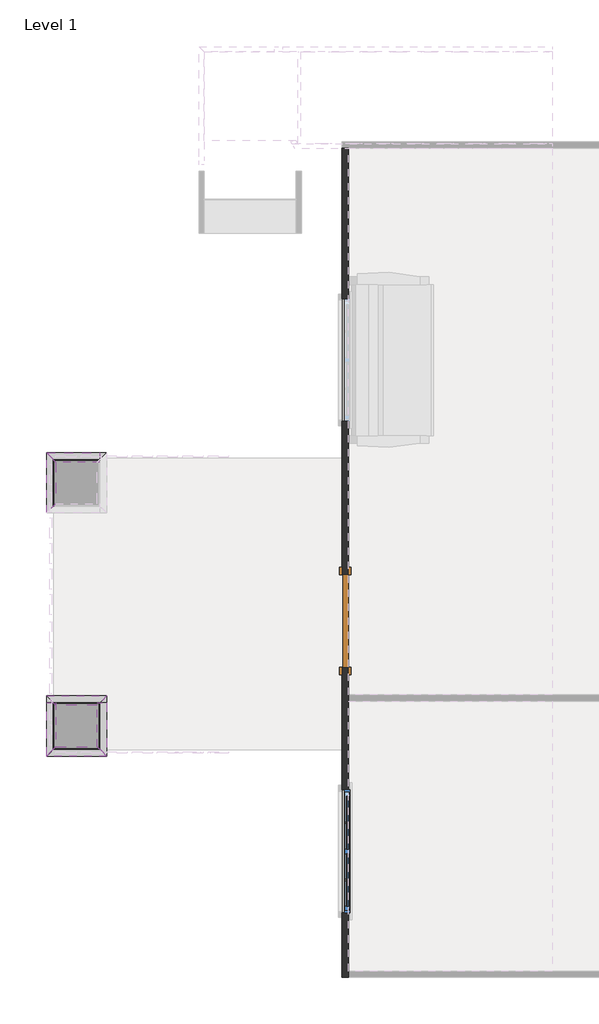
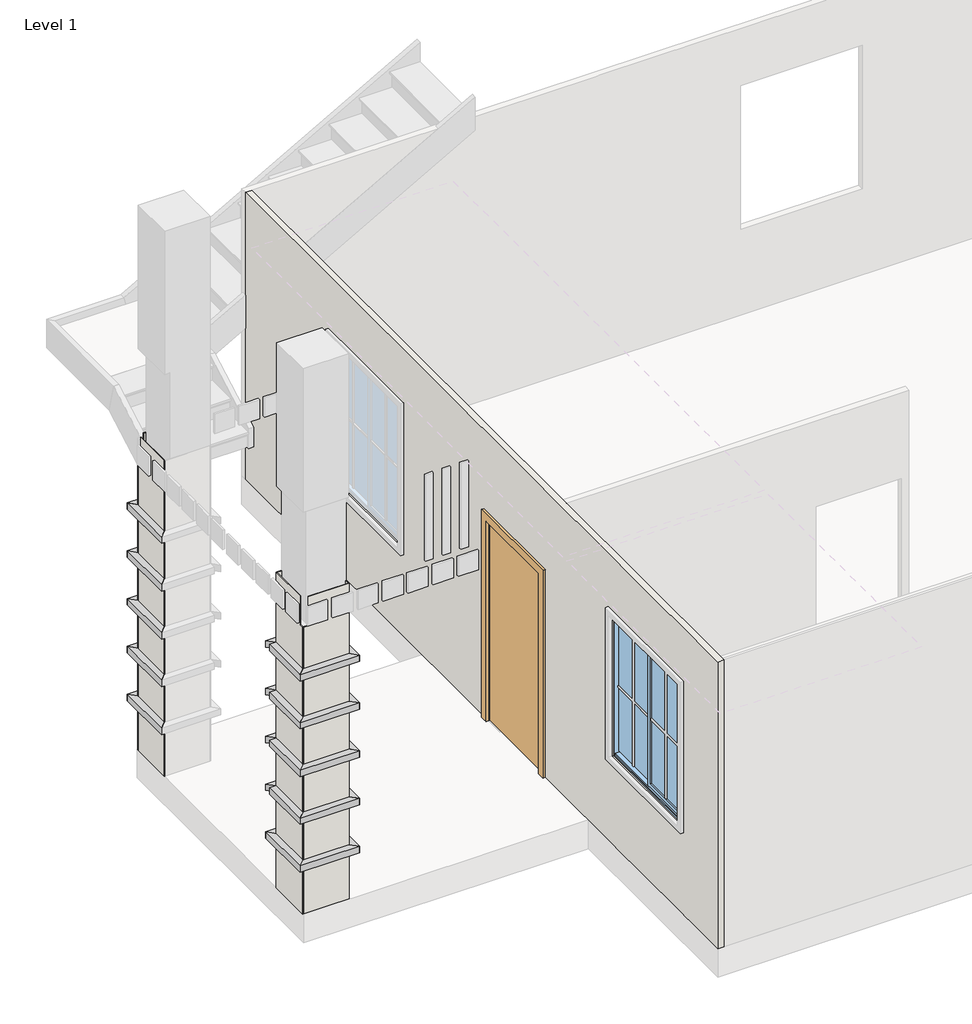
# One storey, part 1 of 3: 31 proxies, 7 walls, 1 door, 1 window.
"""IFC4 building model written with IfcOpenShell, lengths in millimetres."""

import ifcopenshell
import ifcopenshell.guid

model = None  # the IFC model being written
_history = None  # IfcOwnerHistory: only IFC2X3 demands one
_inside = {}  # id of a spatial element -> (the spatial element, [elements in it])
_under = {}  # id of a project, library or spatial element -> (it, [spatial elements below it])
_declared = {}  # id of a project -> (the project, [libraries it declares])
_typed = {}  # id of a type object -> (the type object, [elements of that type])
_made_of = {}  # id of a material, layer set ... -> (it, [elements and type objects made of it])


def new_model(schema):
    """Start an empty IFC model of exactly this schema.

    Asked for "IFC4X3", IfcOpenShell would pick the latest addendum, in which some entities
    have other attributes; the version numbers below select the first issue.
    IFC2X3 requires an IfcOwnerHistory on every rooted entity: one is made here for all.
    """
    global model, _history
    if schema == "IFC4X3":
        model = ifcopenshell.file(schema_version=(4, 3, 0, 0))
    else:
        model = ifcopenshell.file(schema=schema)
    _inside.clear()
    _under.clear()
    _declared.clear()
    _typed.clear()
    _made_of.clear()
    _history = None
    if model.schema == "IFC2X3":
        org = make("IfcOrganization", Name="unknown")
        user = make(
            "IfcPersonAndOrganization",
            ThePerson=make("IfcPerson", FamilyName="unknown"),
            TheOrganization=org,
        )
        app = make(
            "IfcApplication",
            ApplicationDeveloper=org,
            Version="unknown",
            ApplicationFullName="unknown",
            ApplicationIdentifier="unknown",
        )
        _history = make(
            "IfcOwnerHistory",
            OwningUser=user,
            OwningApplication=app,
            ChangeAction="ADDED",
            CreationDate=0,
        )
    return model


def make(cls, **values):
    """One entity of the class cls with the attributes given. An attribute that is None is left unset."""
    return model.create_entity(
        cls, **{name: value for name, value in values.items() if value is not None}
    )


def rooted(cls, **values):
    """An entity with a GlobalId (a new one), such as an element, a storey or a relation."""
    return make(cls, GlobalId=ifcopenshell.guid.new(), OwnerHistory=_history, **values)


def si_unit(unit_type, name, prefix=None):
    """IfcSIUnit, for example si_unit("LENGTHUNIT", "METRE", prefix="MILLI")."""
    return make("IfcSIUnit", UnitType=unit_type, Prefix=prefix, Name=name)


def assignment(units):
    """IfcUnitAssignment: the units of a project."""
    return None if units is None else make("IfcUnitAssignment", Units=units)


def point(xyz):
    """IfcCartesianPoint."""
    return None if xyz is None else make("IfcCartesianPoint", Coordinates=xyz)


def direction(xyz):
    """IfcDirection."""
    return None if xyz is None else make("IfcDirection", DirectionRatios=xyz)


def frame(location, z_axis=None, x_axis=None):
    """IfcAxis2Placement3D, a coordinate frame: its origin and axes. An axis left out is left unset."""
    return make(
        "IfcAxis2Placement3D",
        Location=point(location),
        Axis=direction(z_axis),
        RefDirection=direction(x_axis),
    )


def origin():
    """The frame at (0, 0, 0) with its axes left unset."""
    return frame((0.0, 0.0, 0.0))


def origin_with_axes():
    """The frame at (0, 0, 0) with the z axis (0, 0, 1) and the x axis (1, 0, 0) written out."""
    return frame((0.0, 0.0, 0.0), z_axis=(0.0, 0.0, 1.0), x_axis=(1.0, 0.0, 0.0))


def place(relative_to, where):
    """IfcLocalPlacement: puts the frame where relative to a parent placement (None: the world)."""
    return make(
        "IfcLocalPlacement", PlacementRelTo=relative_to, RelativePlacement=where
    )


def context(
    kind, dimensions, precision=None, world=None, true_north=None, identifier=None
):
    """IfcGeometricRepresentationContext, for example the 3D "Model" context."""
    return make(
        "IfcGeometricRepresentationContext",
        ContextIdentifier=identifier,
        ContextType=kind,
        CoordinateSpaceDimension=dimensions,
        Precision=precision,
        WorldCoordinateSystem=world,
        TrueNorth=true_north,
    )


def project(units=None, contexts=None):
    """IfcProject with its units and contexts."""
    return rooted(
        "IfcProject",
        Name="project",
        RepresentationContexts=contexts,
        UnitsInContext=assignment(units),
    )


def spatial(cls, under=None, at=None, **own):
    """A site, building, storey or space (cls), placed at a placement, below another one or the project."""
    s = rooted(cls, ObjectPlacement=at, **own)
    if under is not None:
        _under.setdefault(under.id(), (under, []))[1].append(s)
    return s


def polyline(points):
    """IfcPolyline through the points."""
    return make("IfcPolyline", Points=[point(p) for p in points])


def outline(outer, holes=None, kind="AREA"):
    """IfcArbitraryClosedProfileDef: a profile drawn as a closed curve; with holes, ...WithVoids."""
    if holes is None:
        return make("IfcArbitraryClosedProfileDef", ProfileType=kind, OuterCurve=outer)
    return make(
        "IfcArbitraryProfileDefWithVoids",
        ProfileType=kind,
        OuterCurve=outer,
        InnerCurves=holes,
    )


def extrude(swept, where, along, depth):
    """IfcExtrudedAreaSolid: the profile swept, set in the frame where, extruded along a direction by depth."""
    return make(
        "IfcExtrudedAreaSolid",
        SweptArea=swept,
        Position=where,
        ExtrudedDirection=direction(along),
        Depth=depth,
    )


def faces_of(points, faces, orient=None, outer=None):
    """IfcFace entities. A face is a list of loops; a loop is a list of indices into points, from 0.

    orient and outer hold one flag for each loop. By default every Orientation is true, the
    first loop of a face is its IfcFaceOuterBound and the others are IfcFaceBound.
    """
    made = []
    for i, loops in enumerate(faces):
        bounds = []
        for j, loop in enumerate(loops):
            is_outer = j == 0 if outer is None else outer[i][j]
            bounds.append(
                make(
                    "IfcFaceOuterBound" if is_outer else "IfcFaceBound",
                    Bound=make("IfcPolyLoop", Polygon=[points[k] for k in loop]),
                    Orientation=True if orient is None else orient[i][j],
                )
            )
        made.append(make("IfcFace", Bounds=bounds))
    return made


def faceted_brep(points, faces, orient=None, outer=None, voids=None):
    """IfcFacetedBrep: a solid bounded by flat faces; with voids (closed shells), ...WithVoids."""
    shared = [point(p) for p in points]
    hull = make("IfcClosedShell", CfsFaces=faces_of(shared, faces, orient, outer))
    if voids is None:
        return make("IfcFacetedBrep", Outer=hull)
    return make(
        "IfcFacetedBrepWithVoids",
        Outer=hull,
        Voids=[
            make(cls, CfsFaces=faces_of(shared, fs, o, b)) for cls, fs, o, b in voids
        ],
    )


def shape(context_of_items, identifier, shape_type, items):
    """IfcShapeRepresentation: the items that make up one representation, for example the "Body"."""
    return make(
        "IfcShapeRepresentation",
        ContextOfItems=context_of_items,
        RepresentationIdentifier=identifier,
        RepresentationType=shape_type,
        Items=items,
    )


def source(mapping_origin, context_of_items, identifier, shape_type, items):
    """IfcRepresentationMap: a shape defined once, which mapped items show again and again."""
    return make(
        "IfcRepresentationMap",
        MappingOrigin=mapping_origin,
        MappedRepresentation=shape(context_of_items, identifier, shape_type, items),
    )


def transform(
    local_origin,
    x_axis=None,
    y_axis=None,
    z_axis=None,
    scale=None,
    scale2=None,
    scale3=None,
    uniform=True,
):
    """IfcCartesianTransformationOperator3D, or its non-uniform kind. x_axis, y_axis, z_axis: its Axis1, 2, 3."""
    if uniform:
        return make(
            "IfcCartesianTransformationOperator3D",
            Axis1=direction(x_axis),
            Axis2=direction(y_axis),
            LocalOrigin=point(local_origin),
            Scale=scale,
            Axis3=direction(z_axis),
        )
    return make(
        "IfcCartesianTransformationOperator3DnonUniform",
        Axis1=direction(x_axis),
        Axis2=direction(y_axis),
        LocalOrigin=point(local_origin),
        Scale=scale,
        Axis3=direction(z_axis),
        Scale2=scale2,
        Scale3=scale3,
    )


def mapped(mapping_source, mapping_target):
    """IfcMappedItem: shows the shape of a source again, moved by a transform."""
    return make(
        "IfcMappedItem", MappingSource=mapping_source, MappingTarget=mapping_target
    )


def made_of(thing, what):
    """Note that an element or type object is made of a material, layer set ...; save() writes the relation."""
    if what is not None:
        _made_of.setdefault(what.id(), (what, []))[1].append(thing)
    return thing


def element(
    cls,
    number,
    at=None,
    inside=None,
    cuts=None,
    type_object=None,
    material=None,
    context=None,
    identifier="Body",
    shape_type=None,
    held_by="IfcProductDefinitionShape",
    body=None,
    shapes=None,
    **own,
):
    """One element of the class cls, such as IfcWall. Its Tag is "e" and its number.

    at: its placement. inside: the storey or other place that contains it. cuts: it is an
    opening in that element (IfcRelVoidsElement). A single representation is given by context,
    identifier, shape_type and body (its items); several are given by shapes. held_by: the class
    of the entity that holds the representations. save() writes the other relations.
    """
    e = rooted(cls, Tag="e%d" % number, ObjectPlacement=at, **own)
    if body is not None:
        shapes = [shape(context, identifier, shape_type, body)]
    if shapes is not None:
        e.Representation = make(held_by, Representations=shapes)
    if inside is not None:
        _inside.setdefault(inside.id(), (inside, []))[1].append(e)
    if cuts is not None:
        rooted(
            "IfcRelVoidsElement", RelatingBuildingElement=cuts, RelatedOpeningElement=e
        )
    if type_object is not None:
        _typed.setdefault(type_object.id(), (type_object, []))[1].append(e)
    return made_of(e, material)


def aggregate(whole, parts):
    """IfcRelAggregates: a whole, such as a stair, and the parts it consists of."""
    return rooted("IfcRelAggregates", RelatingObject=whole, RelatedObjects=parts)


def save(model, path):
    """Write the relations noted so far, then the file.

    IfcRelAggregates (storeys below a building ...), IfcRelContainedInSpatialStructure (elements
    in a storey), IfcRelDefinesByType, IfcRelAssociatesMaterial and IfcRelDeclares: one each for
    every whole, place, type object, material and project.
    """
    for whole, parts in _under.values():
        aggregate(whole, parts)
    for where, things in _inside.values():
        rooted(
            "IfcRelContainedInSpatialStructure",
            RelatedElements=things,
            RelatingStructure=where,
        )
    for kind, things in _typed.values():
        rooted("IfcRelDefinesByType", RelatedObjects=things, RelatingType=kind)
    for what, things in _made_of.values():
        rooted("IfcRelAssociatesMaterial", RelatedObjects=things, RelatingMaterial=what)
    for by, libraries in _declared.values():
        rooted("IfcRelDeclares", RelatingContext=by, RelatedDefinitions=libraries)
    model.write(path)


def door_5bbd86ef(model_context):
    return source(origin(), model_context, "Body", "SweptSolid", [
        extrude(outline(polyline([(2209.8, -533.4), (0.0, -533.4), (0.0, -457.2), (2133.6, -457.2), (2133.6, 457.2), (0.0, 457.2), (0.0, 533.4), (2209.8, 533.4), (2209.8, -533.4)])), frame((0.0, 31.75, 0.0), z_axis=(0.0, 1.0, 0.0), x_axis=(0.0, 0.0, 1.0)), (0.0, 0.0, 1.0), 25.4),
        extrude(outline(polyline([(2209.8, 533.4), (2209.8, -533.4), (0.0, -533.4), (0.0, -457.2), (2133.6, -457.2), (2133.6, 457.2), (0.0, 457.2), (0.0, 533.4), (2209.8, 533.4)])), frame((0.0, -57.15, 0.0), z_axis=(0.0, 1.0, 0.0), x_axis=(0.0, 0.0, 1.0)), (0.0, 0.0, 1.0), 25.4),
        extrude(outline(polyline([(457.2, -19.05), (-457.2, -19.05), (-457.2, 31.75), (457.2, 31.75), (457.2, -19.05)])), origin_with_axes(), (0.0, 0.0, 1.0), 2133.6),
    ])


def window_57c2f901(model_context):
    return source(origin(), model_context, "Body", "SolidModel", [
        faceted_brep([(-609.6, -10.16, 914.4), (-609.6, 46.99, 914.4), (609.6, 46.99, 914.4), (609.6, -10.16, 914.4), (-568.6778905, 46.99, 2397.4778905), (-568.6778905, 40.64, 2397.4778905), (-568.6778905, 40.64, 952.5), (-568.6778905, 40.64, 933.45), (-568.6778905, 46.99, 933.45), (568.6778905, 40.64, 2397.4778905), (568.6778905, 40.64, 952.5), (590.55, 40.64, 952.5), (590.55, 40.64, 2419.35), (-590.55, 40.64, 2419.35), (-590.55, 40.64, 952.5), (-590.55, -10.16, 2419.35), (-590.55, -10.16, 933.45), (-590.55, -3.81, 933.45), (-590.55, -3.81, 952.5), (609.6, -10.16, 2438.4), (-609.6, -10.16, 2438.4), (590.55, -10.16, 2419.35), (590.55, -10.16, 933.45), (-609.6, 46.99, 2438.4), (609.6, 46.99, 2438.4), (568.6778905, 46.99, 933.45), (568.6778905, 46.99, 2397.4778905), (568.6778905, 40.64, 933.45), (590.55, -3.81, 952.5), (590.55, -3.81, 933.45)], [[[0, 1, 2, 3]], [[4, 5, 6, 7, 8]], [[5, 9, 10, 11, 12, 13, 14, 6]], [[13, 15, 16, 17, 18, 14]], [[0, 3, 19, 20], [21, 22, 16, 15]], [[23, 1, 0, 20]], [[2, 1, 23, 24], [4, 8, 25, 26]], [[5, 4, 26, 9]], [[13, 12, 21, 15]], [[20, 19, 24, 23]], [[9, 26, 25, 27, 10]], [[21, 12, 11, 28, 29, 22]], [[19, 3, 2, 24]], [[7, 27, 25, 8]], [[27, 7, 6, 10]], [[10, 6, 14, 18, 28, 11]], [[28, 18, 17, 29]], [[16, 22, 29, 17]]]),
        extrude(outline(polyline([(546.1, 27.94), (546.1, 21.59), (22.225, 21.59), (22.225, 27.94), (546.1, 27.94)])), frame((0.0, 0.0, 996.95), z_axis=(0.0, 0.0, 1.0), x_axis=(1.0, 0.0, 0.0)), (0.0, 0.0, 1.0), 1377.95),
        extrude(outline(polyline([(546.1, 15.24), (546.1, 8.89), (22.225, 8.89), (22.225, 15.24), (546.1, 15.24)])), frame((0.0, 0.0, 996.95), z_axis=(0.0, 0.0, 1.0), x_axis=(1.0, 0.0, 0.0)), (0.0, 0.0, 1.0), 1377.95),
        extrude(outline(polyline([(-22.225, 27.94), (-22.225, 21.59), (-546.1, 21.59), (-546.1, 27.94), (-22.225, 27.94)])), frame((0.0, 0.0, 996.95), z_axis=(0.0, 0.0, 1.0), x_axis=(1.0, 0.0, 0.0)), (0.0, 0.0, 1.0), 1377.95),
        extrude(outline(polyline([(-22.225, 15.24), (-22.225, 8.89), (-546.1, 8.89), (-546.1, 15.24), (-22.225, 15.24)])), frame((0.0, 0.0, 996.95), z_axis=(0.0, 0.0, 1.0), x_axis=(1.0, 0.0, 0.0)), (0.0, 0.0, 1.0), 1377.95),
        extrude(outline(polyline([(952.5, 590.55), (2419.35, 590.55), (2419.35, -22.225), (952.5, -22.225), (952.5, 590.55)]), holes=[polyline([(996.95, 22.225), (2374.9, 22.225), (2374.9, 546.1), (996.95, 546.1), (996.95, 22.225)])]), frame((0.0, -3.81, 0.0), z_axis=(0.0, 1.0, 0.0), x_axis=(0.0, 0.0, 1.0)), (0.0, 0.0, 1.0), 44.45),
    ])


model = new_model("IFC4")

# Units and contexts
model_context = context("Model", 3, world=origin())
ifc_project = project(units=[si_unit("LENGTHUNIT", "METRE", prefix="MILLI")], contexts=[model_context])

# Site, building, storey
site = spatial("IfcSite", under=ifc_project)
building = spatial("IfcBuilding", under=site)
storey = spatial("IfcBuildingStorey", under=building, Name="Level 1", Elevation=0.0)

# Proxies
placement = place(None, origin())
element("IfcBuildingElementProxy", 1, Name="Reveal", ObjectType="Reveal", at=placement, inside=storey, context=model_context, shape_type="SweptSolid", body=[
    extrude(outline(polyline([(-11412.6148468, 4103.0208836), (-11320.5398468, 4103.0208836), (-11320.5398468, 3664.8708836), (-11412.6148468, 3572.7958836), (-11412.6148468, 4103.0208836)])), frame((0.0, 0.0, 2540.0), z_axis=(0.0, 0.0, 1.0), x_axis=(1.0, 0.0, 0.0)), (0.0, 0.0, 1.0), 67.7333333),
])
element("IfcBuildingElementProxy", 2, Name="Reveal", ObjectType="Reveal", at=placement, inside=storey, context=model_context, shape_type="SweptSolid", body=[
    extrude(outline(polyline([(-11412.6148468, 3572.7958836), (-11320.5398468, 3664.8708836), (-10907.7898468, 3664.8708836), (-10815.7148468, 3572.7958836), (-11412.6148468, 3572.7958836)])), frame((0.0, 0.0, 2540.0), z_axis=(0.0, 0.0, 1.0), x_axis=(1.0, 0.0, 0.0)), (0.0, 0.0, 1.0), 67.7333333),
])
element("IfcBuildingElementProxy", 3, Name="Reveal", ObjectType="Reveal", at=placement, inside=storey, context=model_context, shape_type="SweptSolid", body=[
    extrude(outline(polyline([(-11412.6148468, 4103.0208836), (-11320.5398468, 4103.0208836), (-11320.5398468, 3664.8708836), (-11412.6148468, 3572.7958836), (-11412.6148468, 4103.0208836)])), frame((0.0, 0.0, 2032.0), z_axis=(0.0, 0.0, 1.0), x_axis=(1.0, 0.0, 0.0)), (0.0, 0.0, 1.0), 67.7333333),
])
element("IfcBuildingElementProxy", 4, Name="Reveal", ObjectType="Reveal", at=placement, inside=storey, context=model_context, shape_type="SweptSolid", body=[
    extrude(outline(polyline([(-11412.6148468, 3572.7958836), (-11320.5398468, 3664.8708836), (-10907.7898468, 3664.8708836), (-10815.7148468, 3572.7958836), (-11412.6148468, 3572.7958836)])), frame((0.0, 0.0, 2032.0), z_axis=(0.0, 0.0, 1.0), x_axis=(1.0, 0.0, 0.0)), (0.0, 0.0, 1.0), 67.7333333),
])
element("IfcBuildingElementProxy", 5, Name="Reveal", ObjectType="Reveal", at=placement, inside=storey, context=model_context, shape_type="SweptSolid", body=[
    extrude(outline(polyline([(-11412.6148468, 4103.0208836), (-11320.5398468, 4103.0208836), (-11320.5398468, 3664.8708836), (-11412.6148468, 3572.7958836), (-11412.6148468, 4103.0208836)])), frame((0.0, 0.0, 1524.0), z_axis=(0.0, 0.0, 1.0), x_axis=(1.0, 0.0, 0.0)), (0.0, 0.0, 1.0), 67.7333333),
])
element("IfcBuildingElementProxy", 6, Name="Reveal", ObjectType="Reveal", at=placement, inside=storey, context=model_context, shape_type="SweptSolid", body=[
    extrude(outline(polyline([(-11412.6148468, 3572.7958836), (-11320.5398468, 3664.8708836), (-10907.7898468, 3664.8708836), (-10815.7148468, 3572.7958836), (-11412.6148468, 3572.7958836)])), frame((0.0, 0.0, 1524.0), z_axis=(0.0, 0.0, 1.0), x_axis=(1.0, 0.0, 0.0)), (0.0, 0.0, 1.0), 67.7333333),
])
element("IfcBuildingElementProxy", 7, Name="Reveal", ObjectType="Reveal", at=placement, inside=storey, context=model_context, shape_type="SweptSolid", body=[
    extrude(outline(polyline([(-11412.6148468, 4103.0208836), (-11320.5398468, 4103.0208836), (-11320.5398468, 3664.8708836), (-11412.6148468, 3572.7958836), (-11412.6148468, 4103.0208836)])), frame((0.0, 0.0, 1016.0), z_axis=(0.0, 0.0, 1.0), x_axis=(1.0, 0.0, 0.0)), (0.0, 0.0, 1.0), 67.7333333),
])
element("IfcBuildingElementProxy", 8, Name="Reveal", ObjectType="Reveal", at=placement, inside=storey, context=model_context, shape_type="SweptSolid", body=[
    extrude(outline(polyline([(-11412.6148468, 3572.7958836), (-11320.5398468, 3664.8708836), (-10907.7898468, 3664.8708836), (-10815.7148468, 3572.7958836), (-11412.6148468, 3572.7958836)])), frame((0.0, 0.0, 1524.0), z_axis=(0.0, 0.0, 1.0), x_axis=(1.0, 0.0, 0.0)), (0.0, 0.0, 1.0), 67.7333333),
])
element("IfcBuildingElementProxy", 9, Name="Reveal", ObjectType="Reveal", at=placement, inside=storey, context=model_context, shape_type="SweptSolid", body=[
    extrude(outline(polyline([(-11412.6148468, 3572.7958836), (-11320.5398468, 3664.8708836), (-10907.7898468, 3664.8708836), (-10815.7148468, 3572.7958836), (-11412.6148468, 3572.7958836)])), frame((0.0, 0.0, 1016.0), z_axis=(0.0, 0.0, 1.0), x_axis=(1.0, 0.0, 0.0)), (0.0, 0.0, 1.0), 67.7333333),
])
element("IfcBuildingElementProxy", 10, Name="Reveal", ObjectType="Reveal", at=placement, inside=storey, context=model_context, shape_type="SweptSolid", body=[
    extrude(outline(polyline([(-11412.6148468, 3572.7958836), (-11320.5398468, 3664.8708836), (-10907.7898468, 3664.8708836), (-10815.7148468, 3572.7958836), (-11412.6148468, 3572.7958836)])), frame((0.0, 0.0, 508.0), z_axis=(0.0, 0.0, 1.0), x_axis=(1.0, 0.0, 0.0)), (0.0, 0.0, 1.0), 67.7333333),
])
element("IfcBuildingElementProxy", 11, Name="Reveal", ObjectType="Reveal", at=placement, inside=storey, context=model_context, shape_type="SweptSolid", body=[
    extrude(outline(polyline([(-11412.6148468, 4169.6958836), (-11320.5398468, 4077.6208836), (-11320.5398468, 3664.8708836), (-11412.6148468, 3572.7958836), (-11412.6148468, 4169.6958836)])), frame((0.0, 0.0, 508.0), z_axis=(0.0, 0.0, 1.0), x_axis=(1.0, 0.0, 0.0)), (0.0, 0.0, 1.0), 67.7333333),
])
element("IfcBuildingElementProxy", 12, Name="Reveal", ObjectType="Reveal", at=placement, inside=storey, context=model_context, shape_type="SweptSolid", body=[
    extrude(outline(polyline([(-11412.6148468, 6582.6958836), (-11320.5398468, 6490.6208836), (-11320.5398468, 6077.8708836), (-11412.6148468, 5985.7958836), (-11412.6148468, 6582.6958836)])), frame((0.0, 0.0, 2540.0), z_axis=(0.0, 0.0, 1.0), x_axis=(1.0, 0.0, 0.0)), (0.0, 0.0, 1.0), 67.7333333),
])
element("IfcBuildingElementProxy", 13, Name="Reveal", ObjectType="Reveal", at=placement, inside=storey, context=model_context, shape_type="SweptSolid", body=[
    extrude(outline(polyline([(-11412.6148468, 6582.6958836), (-11320.5398468, 6490.6208836), (-11320.5398468, 6077.8708836), (-11412.6148468, 5985.7958836), (-11412.6148468, 6582.6958836)])), frame((0.0, 0.0, 2032.0), z_axis=(0.0, 0.0, 1.0), x_axis=(1.0, 0.0, 0.0)), (0.0, 0.0, 1.0), 67.7333333),
])
element("IfcBuildingElementProxy", 14, Name="Reveal", ObjectType="Reveal", at=placement, inside=storey, context=model_context, shape_type="SweptSolid", body=[
    extrude(outline(polyline([(-11412.6148468, 6582.6958836), (-11320.5398468, 6490.6208836), (-11320.5398468, 6077.8708836), (-11412.6148468, 5985.7958836), (-11412.6148468, 6582.6958836)])), frame((0.0, 0.0, 1524.0), z_axis=(0.0, 0.0, 1.0), x_axis=(1.0, 0.0, 0.0)), (0.0, 0.0, 1.0), 67.7333333),
])
element("IfcBuildingElementProxy", 15, Name="Reveal", ObjectType="Reveal", at=placement, inside=storey, context=model_context, shape_type="SweptSolid", body=[
    extrude(outline(polyline([(-11412.6148468, 6582.6958836), (-11320.5398468, 6490.6208836), (-11320.5398468, 6077.8708836), (-11412.6148468, 5985.7958836), (-11412.6148468, 6582.6958836)])), frame((0.0, 0.0, 1016.0), z_axis=(0.0, 0.0, 1.0), x_axis=(1.0, 0.0, 0.0)), (0.0, 0.0, 1.0), 67.7333333),
])
element("IfcBuildingElementProxy", 16, Name="Reveal", ObjectType="Reveal", at=placement, inside=storey, context=model_context, shape_type="SweptSolid", body=[
    extrude(outline(polyline([(-11412.6148468, 6582.6958836), (-11320.5398468, 6490.6208836), (-11320.5398468, 6077.8708836), (-11412.6148468, 5985.7958836), (-11412.6148468, 6582.6958836)])), frame((0.0, 0.0, 508.0), z_axis=(0.0, 0.0, 1.0), x_axis=(1.0, 0.0, 0.0)), (0.0, 0.0, 1.0), 67.7333333),
])
element("IfcBuildingElementProxy", 17, Name="Reveal", ObjectType="Reveal", at=placement, inside=storey, context=model_context, shape_type="SweptSolid", body=[
    extrude(outline(polyline([(-10815.7148468, 6582.6958836), (-10907.7898468, 6490.6208836), (-11320.5398468, 6490.6208836), (-11412.6148468, 6582.6958836), (-10815.7148468, 6582.6958836)])), frame((0.0, 0.0, 508.0), z_axis=(0.0, 0.0, 1.0), x_axis=(1.0, 0.0, 0.0)), (0.0, 0.0, 1.0), 67.7333333),
])
element("IfcBuildingElementProxy", 18, Name="Reveal", ObjectType="Reveal", at=placement, inside=storey, context=model_context, shape_type="SweptSolid", body=[
    extrude(outline(polyline([(-10882.3898468, 6582.6958836), (-10882.3898468, 6490.6208836), (-11320.5398468, 6490.6208836), (-11412.6148468, 6582.6958836), (-10882.3898468, 6582.6958836)])), frame((0.0, 0.0, 1016.0), z_axis=(0.0, 0.0, 1.0), x_axis=(1.0, 0.0, 0.0)), (0.0, 0.0, 1.0), 67.7333333),
])
element("IfcBuildingElementProxy", 19, Name="Reveal", ObjectType="Reveal", at=placement, inside=storey, context=model_context, shape_type="SweptSolid", body=[
    extrude(outline(polyline([(-10882.3898468, 6582.6958836), (-10882.3898468, 6490.6208836), (-11320.5398468, 6490.6208836), (-11412.6148468, 6582.6958836), (-10882.3898468, 6582.6958836)])), frame((0.0, 0.0, 1524.0), z_axis=(0.0, 0.0, 1.0), x_axis=(1.0, 0.0, 0.0)), (0.0, 0.0, 1.0), 67.7333333),
])
element("IfcBuildingElementProxy", 20, Name="Reveal", ObjectType="Reveal", at=placement, inside=storey, context=model_context, shape_type="SweptSolid", body=[
    extrude(outline(polyline([(-10882.3898468, 6582.6958836), (-10882.3898468, 6490.6208836), (-11320.5398468, 6490.6208836), (-11412.6148468, 6582.6958836), (-10882.3898468, 6582.6958836)])), frame((0.0, 0.0, 2032.0), z_axis=(0.0, 0.0, 1.0), x_axis=(1.0, 0.0, 0.0)), (0.0, 0.0, 1.0), 67.7333333),
])
element("IfcBuildingElementProxy", 21, Name="Reveal", ObjectType="Reveal", at=placement, inside=storey, context=model_context, shape_type="SweptSolid", body=[
    extrude(outline(polyline([(-10882.3898468, 6582.6958836), (-10882.3898468, 6490.6208836), (-11320.5398468, 6490.6208836), (-11412.6148468, 6582.6958836), (-10882.3898468, 6582.6958836)])), frame((0.0, 0.0, 2540.0), z_axis=(0.0, 0.0, 1.0), x_axis=(1.0, 0.0, 0.0)), (0.0, 0.0, 1.0), 67.7333333),
])
element("IfcBuildingElementProxy", 22, Name="Reveal", ObjectType="Reveal", at=placement, inside=storey, context=model_context, shape_type="SweptSolid", body=[
    extrude(outline(polyline([(-10907.7898468, 4077.6208836), (-10815.7148468, 4169.6958836), (-10815.7148468, 3572.7958836), (-10907.7898468, 3664.8708836), (-10907.7898468, 4077.6208836)])), frame((0.0, 0.0, 508.0), z_axis=(0.0, 0.0, 1.0), x_axis=(1.0, 0.0, 0.0)), (0.0, 0.0, 1.0), 67.7333333),
])
element("IfcBuildingElementProxy", 23, Name="Reveal", ObjectType="Reveal", at=placement, inside=storey, context=model_context, shape_type="SweptSolid", body=[
    extrude(outline(polyline([(-10907.7898468, 4103.0208836), (-10815.7148468, 4103.0208836), (-10815.7148468, 3572.7958836), (-10907.7898468, 3664.8708836), (-10907.7898468, 4103.0208836)])), frame((0.0, 0.0, 1016.0), z_axis=(0.0, 0.0, 1.0), x_axis=(1.0, 0.0, 0.0)), (0.0, 0.0, 1.0), 67.7333333),
])
element("IfcBuildingElementProxy", 24, Name="Reveal", ObjectType="Reveal", at=placement, inside=storey, context=model_context, shape_type="SweptSolid", body=[
    extrude(outline(polyline([(-10907.7898468, 4103.0208836), (-10815.7148468, 4103.0208836), (-10815.7148468, 3572.7958836), (-10907.7898468, 3664.8708836), (-10907.7898468, 4103.0208836)])), frame((0.0, 0.0, 1524.0), z_axis=(0.0, 0.0, 1.0), x_axis=(1.0, 0.0, 0.0)), (0.0, 0.0, 1.0), 67.7333333),
])
element("IfcBuildingElementProxy", 25, Name="Reveal", ObjectType="Reveal", at=placement, inside=storey, context=model_context, shape_type="SweptSolid", body=[
    extrude(outline(polyline([(-10907.7898468, 4103.0208836), (-10815.7148468, 4103.0208836), (-10815.7148468, 3572.7958836), (-10907.7898468, 3664.8708836), (-10907.7898468, 4103.0208836)])), frame((0.0, 0.0, 2032.0), z_axis=(0.0, 0.0, 1.0), x_axis=(1.0, 0.0, 0.0)), (0.0, 0.0, 1.0), 67.7333333),
])
element("IfcBuildingElementProxy", 26, Name="Reveal", ObjectType="Reveal", at=placement, inside=storey, context=model_context, shape_type="SweptSolid", body=[
    extrude(outline(polyline([(-10907.7898468, 4103.0208836), (-10815.7148468, 4103.0208836), (-10815.7148468, 3572.7958836), (-10907.7898468, 3664.8708836), (-10907.7898468, 4103.0208836)])), frame((0.0, 0.0, 2540.0), z_axis=(0.0, 0.0, 1.0), x_axis=(1.0, 0.0, 0.0)), (0.0, 0.0, 1.0), 67.7333333),
])
element("IfcBuildingElementProxy", 27, Name="Reveal", ObjectType="Reveal", at=placement, inside=storey, context=model_context, shape_type="SweptSolid", body=[
    extrude(outline(polyline([(-11320.5398468, 4077.6208836), (-11412.6148468, 4169.6958836), (-10815.7148468, 4169.6958836), (-10907.7898468, 4077.6208836), (-11320.5398468, 4077.6208836)])), frame((0.0, 0.0, 508.0), z_axis=(0.0, 0.0, 1.0), x_axis=(1.0, 0.0, 0.0)), (0.0, 0.0, 1.0), 67.7333333),
])
element("IfcBuildingElementProxy", 28, Name="Reveal", ObjectType="Reveal", at=placement, inside=storey, context=model_context, shape_type="SweptSolid", body=[
    extrude(outline(polyline([(-11320.5398468, 4077.6208836), (-11412.6148468, 4169.6958836), (-10815.7148468, 4169.6958836), (-10907.7898468, 4077.6208836), (-11320.5398468, 4077.6208836)])), frame((0.0, 0.0, 1016.0), z_axis=(0.0, 0.0, 1.0), x_axis=(1.0, 0.0, 0.0)), (0.0, 0.0, 1.0), 67.7333333),
])
element("IfcBuildingElementProxy", 29, Name="Reveal", ObjectType="Reveal", at=placement, inside=storey, context=model_context, shape_type="SweptSolid", body=[
    extrude(outline(polyline([(-11320.5398468, 4077.6208836), (-11412.6148468, 4169.6958836), (-10815.7148468, 4169.6958836), (-10907.7898468, 4077.6208836), (-11320.5398468, 4077.6208836)])), frame((0.0, 0.0, 1524.0), z_axis=(0.0, 0.0, 1.0), x_axis=(1.0, 0.0, 0.0)), (0.0, 0.0, 1.0), 67.7333333),
])
element("IfcBuildingElementProxy", 30, Name="Reveal", ObjectType="Reveal", at=placement, inside=storey, context=model_context, shape_type="SweptSolid", body=[
    extrude(outline(polyline([(-11320.5398468, 4077.6208836), (-11412.6148468, 4169.6958836), (-10815.7148468, 4169.6958836), (-10907.7898468, 4077.6208836), (-11320.5398468, 4077.6208836)])), frame((0.0, 0.0, 2032.0), z_axis=(0.0, 0.0, 1.0), x_axis=(1.0, 0.0, 0.0)), (0.0, 0.0, 1.0), 67.7333333),
])
element("IfcBuildingElementProxy", 31, Name="Reveal", ObjectType="Reveal", at=placement, inside=storey, context=model_context, shape_type="SweptSolid", body=[
    extrude(outline(polyline([(-11320.5398468, 4077.6208836), (-11412.6148468, 4169.6958836), (-10815.7148468, 4169.6958836), (-10907.7898468, 4077.6208836), (-11320.5398468, 4077.6208836)])), frame((0.0, 0.0, 2540.0), z_axis=(0.0, 0.0, 1.0), x_axis=(1.0, 0.0, 0.0)), (0.0, 0.0, 1.0), 67.7333333),
])

# Door
door_shape = door_5bbd86ef(model_context)
element("IfcDoor", 32, ObjectType="Single-Flush : 36\" x 84\"", at=placement, inside=storey, context=model_context, shape_type="MappedRepresentation", body=[
    mapped(door_shape, transform((-8447.1648468, 4912.6458836, 0.0), x_axis=(0.0, -1.0, 0.0), y_axis=(1.0, 0.0, 0.0), z_axis=(0.0, 0.0, 1.0))),
])

# Walls
element("IfcWall", 33, ObjectType="pillarhost", at=placement, inside=storey, context=model_context, shape_type="Brep", body=[
    faceted_brep([(-11345.9398468, 4103.0208836, 0.0), (-11345.9398468, 3639.4708836, 0.0), (-11345.9398468, 3639.4708836, 508.0), (-11345.9398468, 4103.0208836, 508.0), (-11339.5898468, 3639.4708836, 0.0), (-11339.5898468, 3645.8208836, 0.0), (-11339.5898468, 4096.6708836, 0.0), (-11339.5898468, 4103.0208836, 0.0), (-11339.5898468, 4103.0208836, 508.0), (-11339.5898468, 4096.6708836, 508.0), (-11339.5898468, 3645.8208836, 508.0), (-11339.5898468, 3639.4708836, 508.0)], [[[0, 1, 2, 3]], [[4, 5, 6, 7, 8, 9, 10, 11]], [[1, 0, 7, 6, 5, 4]], [[1, 4, 11, 2]], [[3, 2, 11, 10, 9, 8]], [[7, 0, 3, 8]]]),
    faceted_brep([(-11345.9398468, 3687.0958836, 3352.8), (-11345.9398468, 4103.0208836, 3352.8), (-11345.9398468, 4103.0208836, 2607.7333333), (-11345.9398468, 3639.4708836, 2607.7333333), (-11345.9398468, 3639.4708836, 3048.0), (-11345.9398468, 3687.0958836, 3048.0), (-11339.5898468, 4103.0208836, 3352.8), (-11339.5898468, 4096.6708836, 3352.8), (-11339.5898468, 3687.0958836, 3352.8), (-11339.5898468, 3687.0958836, 3048.0), (-11339.5898468, 3645.8208836, 3048.0), (-11339.5898468, 3639.4708836, 3048.0), (-11339.5898468, 3639.4708836, 2607.7333333), (-11339.5898468, 3645.8208836, 2607.7333333), (-11339.5898468, 4096.6708836, 2607.7333333), (-11339.5898468, 4103.0208836, 2607.7333333)], [[[0, 1, 2, 3, 4, 5]], [[6, 7, 8, 9, 10, 11, 12, 13, 14, 15]], [[1, 0, 8, 7, 6]], [[5, 4, 11, 10, 9]], [[11, 4, 3, 12]], [[8, 0, 5, 9]], [[12, 3, 2, 15, 14, 13]], [[1, 6, 15, 2]]]),
    faceted_brep([(-11345.9398468, 3639.4708836, 2540.0), (-11345.9398468, 4103.0208836, 2540.0), (-11345.9398468, 4103.0208836, 2099.7333333), (-11345.9398468, 3639.4708836, 2099.7333333), (-11339.5898468, 4103.0208836, 2540.0), (-11339.5898468, 4096.6708836, 2540.0), (-11339.5898468, 3645.8208836, 2540.0), (-11339.5898468, 3639.4708836, 2540.0), (-11339.5898468, 3639.4708836, 2099.7333333), (-11339.5898468, 3645.8208836, 2099.7333333), (-11339.5898468, 4096.6708836, 2099.7333333), (-11339.5898468, 4103.0208836, 2099.7333333)], [[[0, 1, 2, 3]], [[4, 5, 6, 7, 8, 9, 10, 11]], [[7, 0, 3, 8]], [[1, 0, 7, 6, 5, 4]], [[3, 2, 11, 10, 9, 8]], [[1, 4, 11, 2]]]),
    faceted_brep([(-11345.9398468, 3639.4708836, 2032.0), (-11345.9398468, 4103.0208836, 2032.0), (-11345.9398468, 4103.0208836, 1591.7333333), (-11345.9398468, 3639.4708836, 1591.7333333), (-11339.5898468, 4103.0208836, 2032.0), (-11339.5898468, 4096.6708836, 2032.0), (-11339.5898468, 3645.8208836, 2032.0), (-11339.5898468, 3639.4708836, 2032.0), (-11339.5898468, 3639.4708836, 1591.7333333), (-11339.5898468, 3645.8208836, 1591.7333333), (-11339.5898468, 4096.6708836, 1591.7333333), (-11339.5898468, 4103.0208836, 1591.7333333)], [[[0, 1, 2, 3]], [[4, 5, 6, 7, 8, 9, 10, 11]], [[7, 0, 3, 8]], [[1, 0, 7, 6, 5, 4]], [[3, 2, 11, 10, 9, 8]], [[1, 4, 11, 2]]]),
    faceted_brep([(-11345.9398468, 3639.4708836, 1524.0), (-11345.9398468, 4103.0208836, 1524.0), (-11345.9398468, 4103.0208836, 1083.7333333), (-11345.9398468, 3639.4708836, 1083.7333333), (-11339.5898468, 4103.0208836, 1524.0), (-11339.5898468, 4096.6708836, 1524.0), (-11339.5898468, 3645.8208836, 1524.0), (-11339.5898468, 3639.4708836, 1524.0), (-11339.5898468, 3639.4708836, 1083.7333333), (-11339.5898468, 3645.8208836, 1083.7333333), (-11339.5898468, 4096.6708836, 1083.7333333), (-11339.5898468, 4103.0208836, 1083.7333333)], [[[0, 1, 2, 3]], [[4, 5, 6, 7, 8, 9, 10, 11]], [[7, 0, 3, 8]], [[1, 0, 7, 6, 5, 4]], [[3, 2, 11, 10, 9, 8]], [[1, 4, 11, 2]]]),
    faceted_brep([(-11345.9398468, 3639.4708836, 1016.0), (-11345.9398468, 4103.0208836, 1016.0), (-11345.9398468, 4103.0208836, 575.7333333), (-11345.9398468, 3639.4708836, 575.7333333), (-11339.5898468, 4103.0208836, 1016.0), (-11339.5898468, 4096.6708836, 1016.0), (-11339.5898468, 3645.8208836, 1016.0), (-11339.5898468, 3639.4708836, 1016.0), (-11339.5898468, 3639.4708836, 575.7333333), (-11339.5898468, 3645.8208836, 575.7333333), (-11339.5898468, 4096.6708836, 575.7333333), (-11339.5898468, 4103.0208836, 575.7333333)], [[[0, 1, 2, 3]], [[4, 5, 6, 7, 8, 9, 10, 11]], [[7, 0, 3, 8]], [[1, 0, 7, 6, 5, 4]], [[3, 2, 11, 10, 9, 8]], [[1, 4, 11, 2]]]),
])
element("IfcWall", 34, ObjectType="pillarhost", at=placement, inside=storey, context=model_context, shape_type="Brep", body=[
    faceted_brep([(-11339.5898468, 3639.4708836, 0.0), (-10882.3898468, 3639.4708836, 0.0), (-10882.3898468, 3639.4708836, 508.0), (-11339.5898468, 3639.4708836, 508.0), (-10882.3898468, 3645.8208836, 0.0), (-10888.7398468, 3645.8208836, 0.0), (-11339.5898468, 3645.8208836, 0.0), (-11339.5898468, 3645.8208836, 508.0), (-10888.7398468, 3645.8208836, 508.0), (-10882.3898468, 3645.8208836, 508.0)], [[[0, 1, 2, 3]], [[4, 5, 6, 7, 8, 9]], [[1, 0, 6, 5, 4]], [[6, 0, 3, 7]], [[3, 2, 9, 8, 7]], [[1, 4, 9, 2]]]),
    faceted_brep([(-10882.3898468, 3639.4708836, 3352.8), (-11291.6143703, 3639.4708836, 3352.8), (-11291.6143703, 3639.4708836, 3048.0), (-11339.5898468, 3639.4708836, 3048.0), (-11339.5898468, 3639.4708836, 2607.7333333), (-10882.3898468, 3639.4708836, 2607.7333333), (-11291.6143703, 3645.8208836, 3352.8), (-10888.7398468, 3645.8208836, 3352.8), (-10882.3898468, 3645.8208836, 3352.8), (-10882.3898468, 3645.8208836, 2607.7333333), (-10888.7398468, 3645.8208836, 2607.7333333), (-11339.5898468, 3645.8208836, 2607.7333333), (-11339.5898468, 3645.8208836, 3048.0), (-11291.6143703, 3645.8208836, 3048.0)], [[[0, 1, 2, 3, 4, 5]], [[6, 7, 8, 9, 10, 11, 12, 13]], [[1, 0, 8, 7, 6]], [[13, 12, 3, 2]], [[3, 12, 11, 4]], [[1, 6, 13, 2]], [[5, 4, 11, 10, 9]], [[8, 0, 5, 9]]]),
    faceted_brep([(-10882.3898468, 3639.4708836, 2540.0), (-11339.5898468, 3639.4708836, 2540.0), (-11339.5898468, 3639.4708836, 2099.7333333), (-10882.3898468, 3639.4708836, 2099.7333333), (-11339.5898468, 3645.8208836, 2540.0), (-10888.7398468, 3645.8208836, 2540.0), (-10882.3898468, 3645.8208836, 2540.0), (-10882.3898468, 3645.8208836, 2099.7333333), (-10888.7398468, 3645.8208836, 2099.7333333), (-11339.5898468, 3645.8208836, 2099.7333333)], [[[0, 1, 2, 3]], [[4, 5, 6, 7, 8, 9]], [[1, 4, 9, 2]], [[1, 0, 6, 5, 4]], [[3, 2, 9, 8, 7]], [[6, 0, 3, 7]]]),
    faceted_brep([(-10882.3898468, 3639.4708836, 2032.0), (-11339.5898468, 3639.4708836, 2032.0), (-11339.5898468, 3639.4708836, 1591.7333333), (-10882.3898468, 3639.4708836, 1591.7333333), (-11339.5898468, 3645.8208836, 2032.0), (-10888.7398468, 3645.8208836, 2032.0), (-10882.3898468, 3645.8208836, 2032.0), (-10882.3898468, 3645.8208836, 1591.7333333), (-10888.7398468, 3645.8208836, 1591.7333333), (-11339.5898468, 3645.8208836, 1591.7333333)], [[[0, 1, 2, 3]], [[4, 5, 6, 7, 8, 9]], [[1, 4, 9, 2]], [[1, 0, 6, 5, 4]], [[3, 2, 9, 8, 7]], [[6, 0, 3, 7]]]),
    faceted_brep([(-10882.3898468, 3639.4708836, 1524.0), (-11339.5898468, 3639.4708836, 1524.0), (-11339.5898468, 3639.4708836, 1083.7333333), (-10882.3898468, 3639.4708836, 1083.7333333), (-11339.5898468, 3645.8208836, 1524.0), (-10888.7398468, 3645.8208836, 1524.0), (-10882.3898468, 3645.8208836, 1524.0), (-10882.3898468, 3645.8208836, 1083.7333333), (-10888.7398468, 3645.8208836, 1083.7333333), (-11339.5898468, 3645.8208836, 1083.7333333)], [[[0, 1, 2, 3]], [[4, 5, 6, 7, 8, 9]], [[1, 4, 9, 2]], [[1, 0, 6, 5, 4]], [[3, 2, 9, 8, 7]], [[6, 0, 3, 7]]]),
    faceted_brep([(-10882.3898468, 3639.4708836, 1016.0), (-11339.5898468, 3639.4708836, 1016.0), (-11339.5898468, 3639.4708836, 575.7333333), (-10882.3898468, 3639.4708836, 575.7333333), (-11339.5898468, 3645.8208836, 1016.0), (-10888.7398468, 3645.8208836, 1016.0), (-10882.3898468, 3645.8208836, 1016.0), (-10882.3898468, 3645.8208836, 575.7333333), (-10888.7398468, 3645.8208836, 575.7333333), (-11339.5898468, 3645.8208836, 575.7333333)], [[[0, 1, 2, 3]], [[4, 5, 6, 7, 8, 9]], [[1, 4, 9, 2]], [[1, 0, 6, 5, 4]], [[3, 2, 9, 8, 7]], [[6, 0, 3, 7]]]),
])
element("IfcWall", 35, ObjectType="pillarhost", at=placement, inside=storey, context=model_context, shape_type="Brep", body=[
    faceted_brep([(-10882.3898468, 6516.0208836, 0.0), (-11345.9398468, 6516.0208836, 0.0), (-11345.9398468, 6516.0208836, 508.0), (-10882.3898468, 6516.0208836, 508.0), (-11345.9398468, 6509.6708836, 0.0), (-11339.5898468, 6509.6708836, 0.0), (-10888.7398468, 6509.6708836, 0.0), (-10882.3898468, 6509.6708836, 0.0), (-10882.3898468, 6509.6708836, 508.0), (-10888.7398468, 6509.6708836, 508.0), (-11339.5898468, 6509.6708836, 508.0), (-11345.9398468, 6509.6708836, 508.0)], [[[0, 1, 2, 3]], [[4, 5, 6, 7, 8, 9, 10, 11]], [[1, 0, 7, 6, 5, 4]], [[1, 4, 11, 2]], [[3, 2, 11, 10, 9, 8]], [[7, 0, 3, 8]]]),
    faceted_brep([(-11291.6143703, 6516.0208836, 3352.8), (-10882.3898468, 6516.0208836, 3352.8), (-10882.3898468, 6516.0208836, 2607.7333333), (-11345.9398468, 6516.0208836, 2607.7333333), (-11345.9398468, 6516.0208836, 3048.0), (-11291.6143703, 6516.0208836, 3048.0), (-10882.3898468, 6509.6708836, 3352.8), (-10888.7398468, 6509.6708836, 3352.8), (-11291.6143703, 6509.6708836, 3352.8), (-11291.6143703, 6509.6708836, 3048.0), (-11339.5898468, 6509.6708836, 3048.0), (-11345.9398468, 6509.6708836, 3048.0), (-11345.9398468, 6509.6708836, 2607.7333333), (-11339.5898468, 6509.6708836, 2607.7333333), (-10888.7398468, 6509.6708836, 2607.7333333), (-10882.3898468, 6509.6708836, 2607.7333333)], [[[0, 1, 2, 3, 4, 5]], [[6, 7, 8, 9, 10, 11, 12, 13, 14, 15]], [[1, 0, 8, 7, 6]], [[5, 4, 11, 10, 9]], [[11, 4, 3, 12]], [[8, 0, 5, 9]], [[3, 2, 15, 14, 13, 12]], [[1, 6, 15, 2]]]),
    faceted_brep([(-10882.3898468, 6516.0208836, 575.7333333), (-11345.9398468, 6516.0208836, 575.7333333), (-11345.9398468, 6516.0208836, 1016.0), (-10882.3898468, 6516.0208836, 1016.0), (-11345.9398468, 6509.6708836, 575.7333333), (-11339.5898468, 6509.6708836, 575.7333333), (-10888.7398468, 6509.6708836, 575.7333333), (-10882.3898468, 6509.6708836, 575.7333333), (-10882.3898468, 6509.6708836, 1016.0), (-10888.7398468, 6509.6708836, 1016.0), (-11339.5898468, 6509.6708836, 1016.0), (-11345.9398468, 6509.6708836, 1016.0)], [[[0, 1, 2, 3]], [[4, 5, 6, 7, 8, 9, 10, 11]], [[1, 4, 11, 2]], [[1, 0, 7, 6, 5, 4]], [[3, 2, 11, 10, 9, 8]], [[7, 0, 3, 8]]]),
    faceted_brep([(-10882.3898468, 6516.0208836, 1083.7333333), (-11345.9398468, 6516.0208836, 1083.7333333), (-11345.9398468, 6516.0208836, 1524.0), (-10882.3898468, 6516.0208836, 1524.0), (-11345.9398468, 6509.6708836, 1083.7333333), (-11339.5898468, 6509.6708836, 1083.7333333), (-10888.7398468, 6509.6708836, 1083.7333333), (-10882.3898468, 6509.6708836, 1083.7333333), (-10882.3898468, 6509.6708836, 1524.0), (-10888.7398468, 6509.6708836, 1524.0), (-11339.5898468, 6509.6708836, 1524.0), (-11345.9398468, 6509.6708836, 1524.0)], [[[0, 1, 2, 3]], [[4, 5, 6, 7, 8, 9, 10, 11]], [[1, 4, 11, 2]], [[1, 0, 7, 6, 5, 4]], [[3, 2, 11, 10, 9, 8]], [[7, 0, 3, 8]]]),
    faceted_brep([(-10882.3898468, 6516.0208836, 1591.7333333), (-11345.9398468, 6516.0208836, 1591.7333333), (-11345.9398468, 6516.0208836, 2032.0), (-10882.3898468, 6516.0208836, 2032.0), (-11345.9398468, 6509.6708836, 1591.7333333), (-11339.5898468, 6509.6708836, 1591.7333333), (-10888.7398468, 6509.6708836, 1591.7333333), (-10882.3898468, 6509.6708836, 1591.7333333), (-10882.3898468, 6509.6708836, 2032.0), (-10888.7398468, 6509.6708836, 2032.0), (-11339.5898468, 6509.6708836, 2032.0), (-11345.9398468, 6509.6708836, 2032.0)], [[[0, 1, 2, 3]], [[4, 5, 6, 7, 8, 9, 10, 11]], [[1, 4, 11, 2]], [[1, 0, 7, 6, 5, 4]], [[3, 2, 11, 10, 9, 8]], [[7, 0, 3, 8]]]),
    faceted_brep([(-10882.3898468, 6516.0208836, 2099.7333333), (-11345.9398468, 6516.0208836, 2099.7333333), (-11345.9398468, 6516.0208836, 2540.0), (-10882.3898468, 6516.0208836, 2540.0), (-11345.9398468, 6509.6708836, 2099.7333333), (-11339.5898468, 6509.6708836, 2099.7333333), (-10888.7398468, 6509.6708836, 2099.7333333), (-10882.3898468, 6509.6708836, 2099.7333333), (-10882.3898468, 6509.6708836, 2540.0), (-10888.7398468, 6509.6708836, 2540.0), (-11339.5898468, 6509.6708836, 2540.0), (-11345.9398468, 6509.6708836, 2540.0)], [[[0, 1, 2, 3]], [[4, 5, 6, 7, 8, 9, 10, 11]], [[1, 4, 11, 2]], [[1, 0, 7, 6, 5, 4]], [[3, 2, 11, 10, 9, 8]], [[7, 0, 3, 8]]]),
])
element("IfcWall", 36, ObjectType="pillarhost", at=placement, inside=storey, context=model_context, shape_type="Brep", body=[
    faceted_brep([(-11345.9398468, 6509.6708836, 0.0), (-11345.9398468, 6052.4708836, 0.0), (-11345.9398468, 6052.4708836, 508.0), (-11345.9398468, 6509.6708836, 508.0), (-11339.5898468, 6052.4708836, 0.0), (-11339.5898468, 6058.8208836, 0.0), (-11339.5898468, 6509.6708836, 0.0), (-11339.5898468, 6509.6708836, 508.0), (-11339.5898468, 6058.8208836, 508.0), (-11339.5898468, 6052.4708836, 508.0)], [[[0, 1, 2, 3]], [[4, 5, 6, 7, 8, 9]], [[1, 0, 6, 5, 4]], [[6, 0, 3, 7]], [[1, 4, 9, 2]], [[3, 2, 9, 8, 7]]]),
    faceted_brep([(-11345.9398468, 6052.4708836, 3352.8), (-11345.9398468, 6466.2141758, 3352.8), (-11345.9398468, 6466.2141758, 3048.0), (-11345.9398468, 6509.6708836, 3048.0), (-11345.9398468, 6509.6708836, 2607.7333333), (-11345.9398468, 6052.4708836, 2607.7333333), (-11339.5898468, 6466.2141758, 3352.8), (-11339.5898468, 6058.8208836, 3352.8), (-11339.5898468, 6052.4708836, 3352.8), (-11339.5898468, 6052.4708836, 2607.7333333), (-11339.5898468, 6058.8208836, 2607.7333333), (-11339.5898468, 6509.6708836, 2607.7333333), (-11339.5898468, 6509.6708836, 3048.0), (-11339.5898468, 6466.2141758, 3048.0)], [[[0, 1, 2, 3, 4, 5]], [[6, 7, 8, 9, 10, 11, 12, 13]], [[1, 0, 8, 7, 6]], [[13, 12, 3, 2]], [[3, 12, 11, 4]], [[1, 6, 13, 2]], [[8, 0, 5, 9]], [[5, 4, 11, 10, 9]]]),
    faceted_brep([(-11345.9398468, 6509.6708836, 2540.0), (-11345.9398468, 6509.6708836, 2099.7333333), (-11345.9398468, 6052.4708836, 2099.7333333), (-11345.9398468, 6052.4708836, 2540.0), (-11339.5898468, 6509.6708836, 2099.7333333), (-11339.5898468, 6509.6708836, 2540.0), (-11339.5898468, 6058.8208836, 2540.0), (-11339.5898468, 6052.4708836, 2540.0), (-11339.5898468, 6052.4708836, 2099.7333333), (-11339.5898468, 6058.8208836, 2099.7333333)], [[[0, 1, 2, 3]], [[4, 5, 6, 7, 8, 9]], [[1, 0, 5, 4]], [[7, 3, 2, 8]], [[0, 3, 7, 6, 5]], [[2, 1, 4, 9, 8]]]),
    faceted_brep([(-11345.9398468, 6509.6708836, 2032.0), (-11345.9398468, 6509.6708836, 1591.7333333), (-11345.9398468, 6052.4708836, 1591.7333333), (-11345.9398468, 6052.4708836, 2032.0), (-11339.5898468, 6509.6708836, 1591.7333333), (-11339.5898468, 6509.6708836, 2032.0), (-11339.5898468, 6058.8208836, 2032.0), (-11339.5898468, 6052.4708836, 2032.0), (-11339.5898468, 6052.4708836, 1591.7333333), (-11339.5898468, 6058.8208836, 1591.7333333)], [[[0, 1, 2, 3]], [[4, 5, 6, 7, 8, 9]], [[1, 0, 5, 4]], [[7, 3, 2, 8]], [[0, 3, 7, 6, 5]], [[2, 1, 4, 9, 8]]]),
    faceted_brep([(-11345.9398468, 6509.6708836, 1524.0), (-11345.9398468, 6509.6708836, 1083.7333333), (-11345.9398468, 6052.4708836, 1083.7333333), (-11345.9398468, 6052.4708836, 1524.0), (-11339.5898468, 6509.6708836, 1083.7333333), (-11339.5898468, 6509.6708836, 1524.0), (-11339.5898468, 6058.8208836, 1524.0), (-11339.5898468, 6052.4708836, 1524.0), (-11339.5898468, 6052.4708836, 1083.7333333), (-11339.5898468, 6058.8208836, 1083.7333333)], [[[0, 1, 2, 3]], [[4, 5, 6, 7, 8, 9]], [[1, 0, 5, 4]], [[7, 3, 2, 8]], [[0, 3, 7, 6, 5]], [[2, 1, 4, 9, 8]]]),
    faceted_brep([(-11345.9398468, 6052.4708836, 1016.0), (-11345.9398468, 6509.6708836, 1016.0), (-11345.9398468, 6509.6708836, 575.7333333), (-11345.9398468, 6052.4708836, 575.7333333), (-11339.5898468, 6509.6708836, 1016.0), (-11339.5898468, 6058.8208836, 1016.0), (-11339.5898468, 6052.4708836, 1016.0), (-11339.5898468, 6052.4708836, 575.7333333), (-11339.5898468, 6058.8208836, 575.7333333), (-11339.5898468, 6509.6708836, 575.7333333)], [[[0, 1, 2, 3]], [[4, 5, 6, 7, 8, 9]], [[1, 4, 9, 2]], [[6, 0, 3, 7]], [[1, 0, 6, 5, 4]], [[3, 2, 9, 8, 7]]]),
])
element("IfcWall", 37, ObjectType="pillarhost", at=placement, inside=storey, context=model_context, shape_type="Brep", body=[
    faceted_brep([(-10882.3898468, 4096.6708836, 3352.8), (-10888.7398468, 4096.6708836, 3352.8), (-11291.6143703, 4096.6708836, 3352.8), (-11339.5898468, 4096.6708836, 3352.8), (-11339.5898468, 4096.6708836, 3048.0), (-11339.5898468, 4096.6708836, 2607.7333333), (-10888.7398468, 4096.6708836, 2607.7333333), (-10882.3898468, 4096.6708836, 2607.7333333), (-11339.5898468, 4103.0208836, 3352.8), (-10882.3898468, 4103.0208836, 3352.8), (-10882.3898468, 4103.0208836, 2607.7333333), (-11339.5898468, 4103.0208836, 2607.7333333)], [[[0, 1, 2, 3, 4, 5, 6, 7]], [[8, 9, 10, 11]], [[3, 2, 1, 0, 9, 8]], [[3, 8, 11, 5, 4]], [[9, 0, 7, 10]], [[5, 11, 10, 7, 6]]]),
    faceted_brep([(-11339.5898468, 4096.6708836, 0.0), (-10888.7398468, 4096.6708836, 0.0), (-10882.3898468, 4096.6708836, 0.0), (-10882.3898468, 4096.6708836, 508.0), (-10888.7398468, 4096.6708836, 508.0), (-11339.5898468, 4096.6708836, 508.0), (-10882.3898468, 4103.0208836, 0.0), (-11339.5898468, 4103.0208836, 0.0), (-11339.5898468, 4103.0208836, 508.0), (-10882.3898468, 4103.0208836, 508.0)], [[[0, 1, 2, 3, 4, 5]], [[6, 7, 8, 9]], [[2, 1, 0, 7, 6]], [[7, 0, 5, 8]], [[2, 6, 9, 3]], [[5, 4, 3, 9, 8]]]),
    faceted_brep([(-11339.5898468, 4096.6708836, 575.7333333), (-10888.7398468, 4096.6708836, 575.7333333), (-10882.3898468, 4096.6708836, 575.7333333), (-10882.3898468, 4096.6708836, 1016.0), (-10888.7398468, 4096.6708836, 1016.0), (-11339.5898468, 4096.6708836, 1016.0), (-10882.3898468, 4103.0208836, 575.7333333), (-11339.5898468, 4103.0208836, 575.7333333), (-11339.5898468, 4103.0208836, 1016.0), (-10882.3898468, 4103.0208836, 1016.0)], [[[0, 1, 2, 3, 4, 5]], [[6, 7, 8, 9]], [[7, 0, 5, 8]], [[2, 6, 9, 3]], [[2, 1, 0, 7, 6]], [[8, 5, 4, 3, 9]]]),
    faceted_brep([(-11339.5898468, 4096.6708836, 2032.0), (-11339.5898468, 4096.6708836, 1591.7333333), (-10888.7398468, 4096.6708836, 1591.7333333), (-10882.3898468, 4096.6708836, 1591.7333333), (-10882.3898468, 4096.6708836, 2032.0), (-10888.7398468, 4096.6708836, 2032.0), (-11339.5898468, 4103.0208836, 1591.7333333), (-11339.5898468, 4103.0208836, 2032.0), (-10882.3898468, 4103.0208836, 2032.0), (-10882.3898468, 4103.0208836, 1591.7333333)], [[[0, 1, 2, 3, 4, 5]], [[6, 7, 8, 9]], [[0, 7, 6, 1]], [[3, 9, 8, 4]], [[7, 0, 5, 4, 8]], [[1, 6, 9, 3, 2]]]),
    faceted_brep([(-11339.5898468, 4096.6708836, 1524.0), (-11339.5898468, 4096.6708836, 1083.7333333), (-10888.7398468, 4096.6708836, 1083.7333333), (-10882.3898468, 4096.6708836, 1083.7333333), (-10882.3898468, 4096.6708836, 1524.0), (-10888.7398468, 4096.6708836, 1524.0), (-11339.5898468, 4103.0208836, 1083.7333333), (-11339.5898468, 4103.0208836, 1524.0), (-10882.3898468, 4103.0208836, 1524.0), (-10882.3898468, 4103.0208836, 1083.7333333)], [[[0, 1, 2, 3, 4, 5]], [[6, 7, 8, 9]], [[0, 7, 6, 1]], [[3, 9, 8, 4]], [[7, 0, 5, 4, 8]], [[1, 6, 9, 3, 2]]]),
    faceted_brep([(-10882.3898468, 4096.6708836, 2540.0), (-10888.7398468, 4096.6708836, 2540.0), (-11339.5898468, 4096.6708836, 2540.0), (-11339.5898468, 4096.6708836, 2099.7333333), (-10888.7398468, 4096.6708836, 2099.7333333), (-10882.3898468, 4096.6708836, 2099.7333333), (-11339.5898468, 4103.0208836, 2540.0), (-10882.3898468, 4103.0208836, 2540.0), (-10882.3898468, 4103.0208836, 2099.7333333), (-11339.5898468, 4103.0208836, 2099.7333333)], [[[0, 1, 2, 3, 4, 5]], [[6, 7, 8, 9]], [[2, 6, 9, 3]], [[5, 8, 7, 0]], [[0, 7, 6, 2, 1]], [[3, 9, 8, 5, 4]]]),
])
element("IfcWall", 38, ObjectType="pillarhost", at=placement, inside=storey, context=model_context, shape_type="Brep", body=[
    faceted_brep([(-10888.7398468, 3645.8208836, 3352.8), (-10888.7398468, 3687.0958836, 3352.8), (-10888.7398468, 4096.6708836, 3352.8), (-10888.7398468, 4096.6708836, 2607.7333333), (-10888.7398468, 3645.8208836, 2607.7333333), (-10888.7398468, 3645.8208836, 3048.0), (-10882.3898468, 4096.6708836, 3352.8), (-10882.3898468, 3645.8208836, 3352.8), (-10882.3898468, 3645.8208836, 2607.7333333), (-10882.3898468, 4096.6708836, 2607.7333333)], [[[0, 1, 2, 3, 4, 5]], [[6, 7, 8, 9]], [[2, 1, 0, 7, 6]], [[7, 0, 5, 4, 8]], [[2, 6, 9, 3]], [[4, 3, 9, 8]]]),
    faceted_brep([(-10888.7398468, 4096.6708836, 0.0), (-10888.7398468, 3645.8208836, 0.0), (-10888.7398468, 3645.8208836, 508.0), (-10888.7398468, 4096.6708836, 508.0), (-10882.3898468, 3645.8208836, 0.0), (-10882.3898468, 4096.6708836, 0.0), (-10882.3898468, 4096.6708836, 508.0), (-10882.3898468, 3645.8208836, 508.0)], [[[0, 1, 2, 3]], [[4, 5, 6, 7]], [[1, 0, 5, 4]], [[1, 4, 7, 2]], [[5, 0, 3, 6]], [[3, 2, 7, 6]]]),
    faceted_brep([(-10888.7398468, 4096.6708836, 1083.7333333), (-10888.7398468, 3645.8208836, 1083.7333333), (-10888.7398468, 3645.8208836, 1524.0), (-10888.7398468, 4096.6708836, 1524.0), (-10882.3898468, 3645.8208836, 1083.7333333), (-10882.3898468, 4096.6708836, 1083.7333333), (-10882.3898468, 4096.6708836, 1524.0), (-10882.3898468, 3645.8208836, 1524.0)], [[[0, 1, 2, 3]], [[4, 5, 6, 7]], [[1, 4, 7, 2]], [[5, 0, 3, 6]], [[1, 0, 5, 4]], [[3, 2, 7, 6]]]),
    faceted_brep([(-10888.7398468, 4096.6708836, 1016.0), (-10888.7398468, 4096.6708836, 575.7333333), (-10888.7398468, 3645.8208836, 575.7333333), (-10888.7398468, 3645.8208836, 1016.0), (-10882.3898468, 4096.6708836, 575.7333333), (-10882.3898468, 4096.6708836, 1016.0), (-10882.3898468, 3645.8208836, 1016.0), (-10882.3898468, 3645.8208836, 575.7333333)], [[[0, 1, 2, 3]], [[4, 5, 6, 7]], [[6, 3, 2, 7]], [[1, 0, 5, 4]], [[0, 3, 6, 5]], [[2, 1, 4, 7]]]),
    faceted_brep([(-10888.7398468, 4096.6708836, 1591.7333333), (-10888.7398468, 3645.8208836, 1591.7333333), (-10888.7398468, 3645.8208836, 2032.0), (-10888.7398468, 4096.6708836, 2032.0), (-10882.3898468, 3645.8208836, 1591.7333333), (-10882.3898468, 4096.6708836, 1591.7333333), (-10882.3898468, 4096.6708836, 2032.0), (-10882.3898468, 3645.8208836, 2032.0)], [[[0, 1, 2, 3]], [[4, 5, 6, 7]], [[1, 4, 7, 2]], [[5, 0, 3, 6]], [[1, 0, 5, 4]], [[3, 2, 7, 6]]]),
    faceted_brep([(-10888.7398468, 4096.6708836, 2099.7333333), (-10888.7398468, 3645.8208836, 2099.7333333), (-10888.7398468, 3645.8208836, 2540.0), (-10888.7398468, 4096.6708836, 2540.0), (-10882.3898468, 3645.8208836, 2099.7333333), (-10882.3898468, 4096.6708836, 2099.7333333), (-10882.3898468, 4096.6708836, 2540.0), (-10882.3898468, 3645.8208836, 2540.0)], [[[0, 1, 2, 3]], [[4, 5, 6, 7]], [[1, 4, 7, 2]], [[5, 0, 3, 6]], [[1, 0, 5, 4]], [[3, 2, 7, 6]]]),
])
element("IfcWall", 39, ObjectType="Generic - 8\"", at=placement, inside=storey, context=model_context, shape_type="Brep", body=[
    faceted_brep([(-8415.4148468, 1375.6958836, 0.0), (-8415.4148468, 1439.1958836, 0.0), (-8415.4148468, 4118.8958836, 0.0), (-8415.4148468, 4182.3958836, 0.0), (-8415.4148468, 4455.4458836, 0.0), (-8415.4148468, 4455.4458836, 2133.6), (-8415.4148468, 5369.8458836, 2133.6), (-8415.4148468, 5369.8458836, 0.0), (-8415.4148468, 9605.2958836, 0.0), (-8415.4148468, 9605.2958836, 3048.0), (-8415.4148468, 4182.3958836, 3048.0), (-8415.4148468, 4118.8958836, 3048.0), (-8415.4148468, 1439.1958836, 3048.0), (-8415.4148468, 1375.6958836, 3048.0), (-8415.4148468, 1375.6958836, 1974.85), (-8415.4148468, 1375.6958836, 1905.0), (-8415.4148468, 6893.8458836, 2438.4), (-8415.4148468, 8113.0458836, 2438.4), (-8415.4148468, 8113.0458836, 914.4), (-8415.4148468, 6893.8458836, 914.4), (-8415.4148468, 2017.0458836, 2438.4), (-8415.4148468, 3236.2458836, 2438.4), (-8415.4148468, 3236.2458836, 914.4), (-8415.4148468, 2017.0458836, 914.4), (-8478.9148468, 4455.4458836, 2133.6), (-8478.9148468, 4455.4458836, 0.0), (-8478.9148468, 1375.6958836, 0.0), (-8478.9148468, 1375.6958836, 3048.0), (-8478.9148468, 9605.2958836, 3048.0), (-8478.9148468, 9605.2958836, 1974.85), (-8478.9148468, 9605.2958836, 1905.0), (-8478.9148468, 9605.2958836, 0.0), (-8478.9148468, 5369.8458836, 0.0), (-8478.9148468, 5369.8458836, 2133.6), (-8478.9148468, 6893.8458836, 2438.4), (-8478.9148468, 6893.8458836, 914.4), (-8478.9148468, 8113.0458836, 914.4), (-8478.9148468, 8113.0458836, 2438.4), (-8478.9148468, 2017.0458836, 2438.4), (-8478.9148468, 2017.0458836, 914.4), (-8478.9148468, 3236.2458836, 914.4), (-8478.9148468, 3236.2458836, 2438.4)], [[[0, 1, 2, 3, 4, 5, 6, 7, 8, 9, 10, 11, 12, 13, 14, 15], [16, 17, 18, 19], [20, 21, 22, 23]], [[24, 25, 26, 27, 28, 29, 30, 31, 32, 33], [34, 35, 36, 37], [38, 39, 40, 41]], [[32, 31, 8, 7]], [[26, 25, 4, 3, 2, 1, 0]], [[0, 15, 14, 13, 27, 26]], [[9, 8, 31, 30, 29, 28]], [[5, 4, 25, 24]], [[6, 5, 24, 33]], [[7, 6, 33, 32]], [[35, 34, 16, 19]], [[36, 35, 19, 18]], [[37, 36, 18, 17]], [[34, 37, 17, 16]], [[39, 38, 20, 23]], [[40, 39, 23, 22]], [[41, 40, 22, 21]], [[38, 41, 21, 20]], [[13, 12, 11, 10, 9, 28, 27]]]),
])

# Window
window_shape = window_57c2f901(model_context)
element("IfcWindow", 40, ObjectType="Window-Sliding-Double : 48\" x 60\"", at=placement, inside=storey, context=model_context, shape_type="MappedRepresentation", body=[
    mapped(window_shape, transform((-8443.3548468, 2626.6458836, 0.0), x_axis=(0.0, -1.0, 0.0), y_axis=(1.0, 0.0, 0.0), z_axis=(0.0, 0.0, 1.0))),
])

save(model, "model.ifc")
